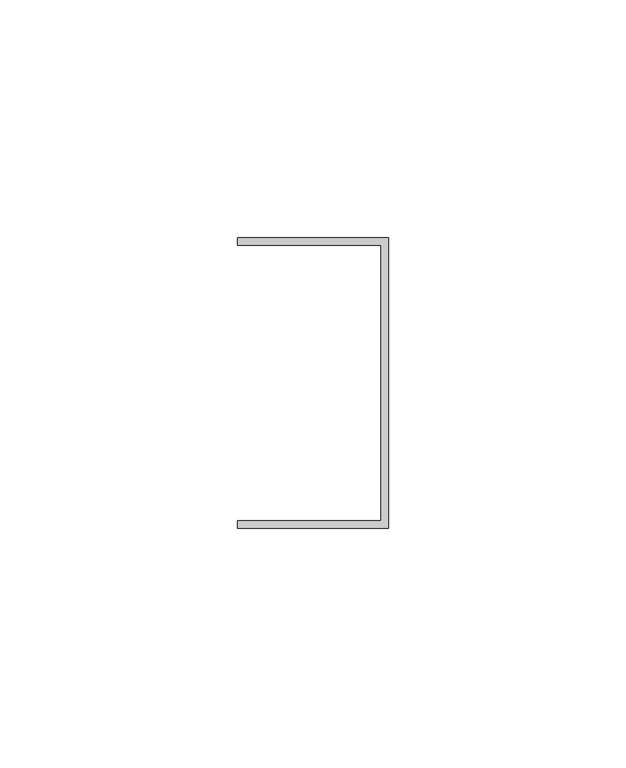
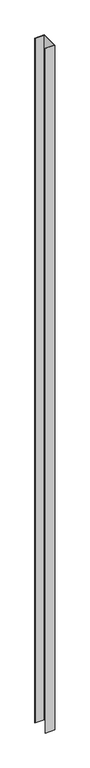
"""IFC4 building model written with IfcOpenShell, lengths in millimetres: proxy geometry, Generic Models 7:Generic Models 1:3:Generic Models 1:3 : Generic Models 7:Generic Models 1:305549:3:Generic Models 1:3:Generic Models 1:3 : Generic Models 7:Generic Models 1:305549:3 : Generic Models 7:Generic Models 1:3:Generic Models 1:3 : Generic Models 7:Generic Models 1:305549:301244:2 : Generic Models 7:Generic Models 1:3:Generic Models 1:3 : Generic Models 7:Generic Models 1:305549:3:Generic Models 1:3:Generic Models 1:3 : Generic Models 7:Generic Models 1:305549:3 : Generic Models 7:Generic Models 1:3:Generic Models 1:3 : Generic Models 7:Generic Models 1:305549:301244:308848."""

from ifc_helpers import new_model, si_unit, frame, origin, place, context, project, spatial, polyline, outline, extrude, source, transform, mapped, element, save


def generic_models_960446eb(model_context):
    return source(origin(), model_context, "Body", "SweptSolid", [
        extrude(outline(polyline([(594938.236724, -579015.772634), (594938.236724, -579076.8913841), (594906.486724, -579076.8913841), (594906.486724, -579075.3038841), (594936.649224, -579075.3038841), (594936.649224, -579017.360134), (594906.486724, -579017.360134), (594906.486724, -579015.772634), (594938.236724, -579015.772634)])), frame((0.0, 0.0, 50.8), z_axis=(0.0, 0.0, 1.0), x_axis=(1.0, 0.0, 0.0)), (0.0, 0.0, 1.0), 2430.9324376),
    ])


if __name__ == "__main__":
    model = new_model("IFC4")
    model_context = context("Model", 3, world=origin())
    ifc_project = project(units=[si_unit("LENGTHUNIT", "METRE", prefix="MILLI")], contexts=[model_context])
    site = spatial("IfcSite", under=ifc_project)
    building = spatial("IfcBuilding", under=site)
    placement = place(None, origin())
    generic_models_shape = generic_models_960446eb(model_context)
    element("IfcBuildingElementProxy", 1, Name="Generic Models 7:Generic Models 1:3:Generic Models 1:3 : Generic Models 7:Generic Models 1:305549:3:Generic Models 1:3:Generic Models 1:3 : Generic Models 7:Generic Models 1:305549:3 : Generic Models 7:Generic Models 1:3:Generic Models 1:3 : Generic Models 7:Generic Models 1:305549:301244:2 : Generic Models 7:Generic Models 1:3:Generic Models 1:3 : Generic Models 7:Generic Models 1:305549:3:Generic Models 1:3:Generic Models 1:3 : Generic Models 7:Generic Models 1:305549:3 : Generic Models 7:Generic Models 1:3:Generic Models 1:3 : Generic Models 7:Generic Models 1:305549:301244:308848", ObjectType="Generic Models 7:Generic Models 1:3:Generic Models 1:3 : Generic Models 7:Generic Models 1:305549:3:Generic Models 1:3:Generic Models 1:3 : Generic Models 7:Generic Models 1:305549:3 : Generic Models 7:Generic Models 1:3:Generic Models 1:3 : Generic Models 7:Generic Models 1:305549:301244:2 : Generic Models 7:Generic Models 1:3:Generic Models 1:3 : Generic Models 7:Generic Models 1:305549:3:Generic Models 1:3:Generic Models 1:3 : Generic Models 7:Generic Models 1:305549:3 : Generic Models 7:Generic Models 1:3:Generic Models 1:3 : Generic Models 7:Generic Models 1:305549:301244:308848", at=placement, inside=building, context=model_context, shape_type="MappedRepresentation", body=[
        mapped(generic_models_shape, transform((0.0, 0.0, 0.0), x_axis=(1.0, 0.0, 0.0), y_axis=(0.0, 1.0, 0.0), z_axis=(0.0, 0.0, 1.0))),
    ])
    save(model, "model.ifc")

# Revit data of these elements
# Type "Generic Models 7:Generic Models 1:3:Generic Models 1:3 : Generic Models 7:Generic Models 1:305549:3:Generic Models 1:3:Generic Models 1:3 : Generic Models 7:Generic Models 1:305549:3 : Generic Models 7:Generic Models 1:3:Generic Models 1:3 : Generic Models 7:Generic Models 1:305549:301244:2 : Generic Models 7:Generic Models 1:3:Generic Models 1:3 : Generic Models 7:Generic Models 1:305549:3:Generic Models 1:3:Generic Models 1:3 : Generic Models 7:Generic Models 1:305549:3 : Generic Models 7:Generic Models 1:3:Generic Models 1:3 : Generic Models 7:Generic Models 1:305549:301244:308848"
#   NameOverride = "Generic Models 7:Generic Models 1:3:Generic Models 1:3 : Generic Models 7:Generic Models 1:305549:3:Generic Models 1:3:Generic Models 1:3 : Generic Models 7:Generic Models 1:305549:3 : Generic Models 7:Generic Models 1:3:Generic Models 1:3 : Generic Models 7:Generic Models 1:305549:301244:308848"
#   ObjectTypeOverride = "Generic Models 1:3:Generic Models 1:3 : Generic Models 7:Generic Models 1:305549:3 : Generic Models 7:Generic Models 1:3:Generic Models 1:3 : Generic Models 7:Generic Models 1:305549:301244"
#   Reference = "Generic Models 1"
#   Tag = "308848"
# Element 1 (IfcBuildingElementProxy, "Generic Models 7:Generic Models 1:3:Generic Models 1:3 : Generic Models 7:Generic Models 1:305549:3:Generic Models 1:3:Generic Models 1:3 : Generic Models 7:Generic Models 1:305549:3 : Generic Models 7:Generic Models 1:3:Generic Models 1:3 : Generic Models 7:Generic Models 1:305549:301244:2 : Generic Models 7:Generic Models 1:3:Generic Models 1:3 : Generic Models 7:Generic Models 1:305549:3:Generic Models 1:3:Generic Models 1:3 : Generic Models 7:Generic Models 1:305549:3 : Generic Models 7:Generic Models 1:3:Generic Models 1:3 : Generic Models 7:Generic Models 1:305549:301244:308848")
#   Materials on its faces: "GALVANIZED U-CHANNEL (250T125-33)"
# Materials
#   "GALVANIZED U-CHANNEL (250T125-33)": class "Unassigned", colour RGB 202 201 200, transparency 0, Keynote = "M05451300.02", Cost = 0
